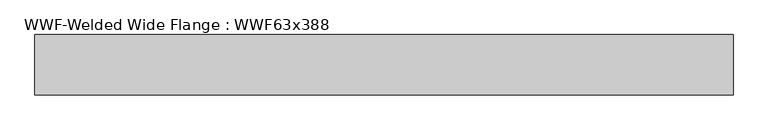
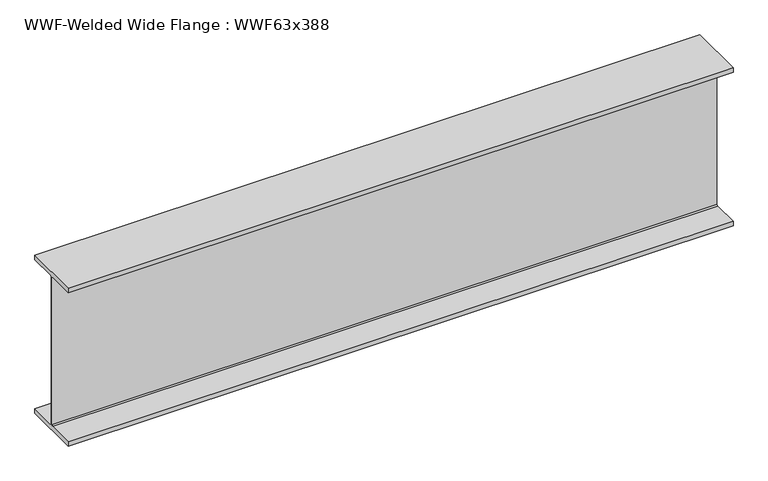
"""IFC4 building model written with IfcOpenShell, lengths in millimetres: beam geometry, WWF-Welded Wide Flange : WWF63x388."""

from ifc_helpers import new_model, si_unit, frame, origin, place, context, project, spatial, polyline, outline, extrude, source, transform, mapped, element, save


def wwf_welded_wide_flange_wwf63x388_45f75be3(model_context):
    return source(origin(), model_context, "Body", "SweptSolid", [
        extrude(outline(polyline([(274.955, -755.015), (274.955, -799.973), (-274.955, -799.973), (-274.955, -755.015), (-19.05, -755.015), (-8.001, -743.966), (-8.001, 743.966), (-19.05, 755.015), (-274.955, 755.015), (-274.955, 799.973), (274.955, 799.973), (274.955, 755.015), (19.05, 755.015), (8.001, 743.966), (8.001, -743.966), (19.05, -755.015), (274.955, -755.015)])), frame((-3184.5840776, 0.0, 0.0), z_axis=(1.0, 0.0, 0.0), x_axis=(0.0, 1.0, 0.0)), (0.0, 0.0, 1.0), 6369.1344444),
    ])


if __name__ == "__main__":
    model = new_model("IFC4")
    model_context = context("Model", 3, world=origin())
    ifc_project = project(units=[si_unit("LENGTHUNIT", "METRE", prefix="MILLI")], contexts=[model_context])
    site = spatial("IfcSite", under=ifc_project)
    building = spatial("IfcBuilding", under=site)
    placement = place(None, origin())
    wwf_welded_wide_flange_wwf63x388_shape = wwf_welded_wide_flange_wwf63x388_45f75be3(model_context)
    element("IfcBeam", 1, ObjectType="WWF-Welded Wide Flange : WWF63x388", at=placement, inside=building, context=model_context, shape_type="MappedRepresentation", body=[
        mapped(wwf_welded_wide_flange_wwf63x388_shape, transform((0.0, 0.0, 0.0), x_axis=(1.0, 0.0, 0.0), y_axis=(0.0, 1.0, 0.0), z_axis=(0.0, 0.0, 1.0))),
    ])
    save(model, "model.ifc")

# Revit data of these elements
# Type "WWF-Welded Wide Flange : WWF63x388"
#   Assembly Code = "B10"
#   Nominal d = "12"
#   W = 388
#   Length [instance default] = 1524 mm
#   bf = 549.91 mm
#   d = 1599.946 mm
#   k = 19.05 mm
#   tf = 44.958 mm
#   tw = 16.002 mm
#   A = 0.0735482 m²
#   Structural Material [instance default] = Steel ASTM A572
# Element 1 (IfcBeam, "WWF-Welded Wide Flange : WWF63x388")
#   Structural Material = Metal - Steel 43-275
#   Materials on its faces: "Metal - Steel 43-275"
# Materials
#   "Steel ASTM A572": class "Metal", colour RGB 247 247 247, transparency 0, Description = "Structural steel, high strength low alloy, ASTM - A572 - 50", Cost = 0
#   "Metal - Steel 43-275": class "Metal", colour RGB 247 247 247, transparency 0, Cost = 0
